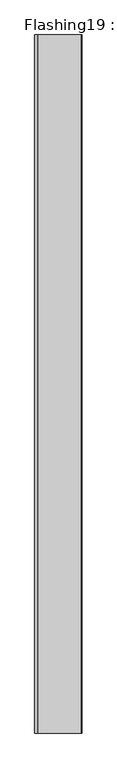
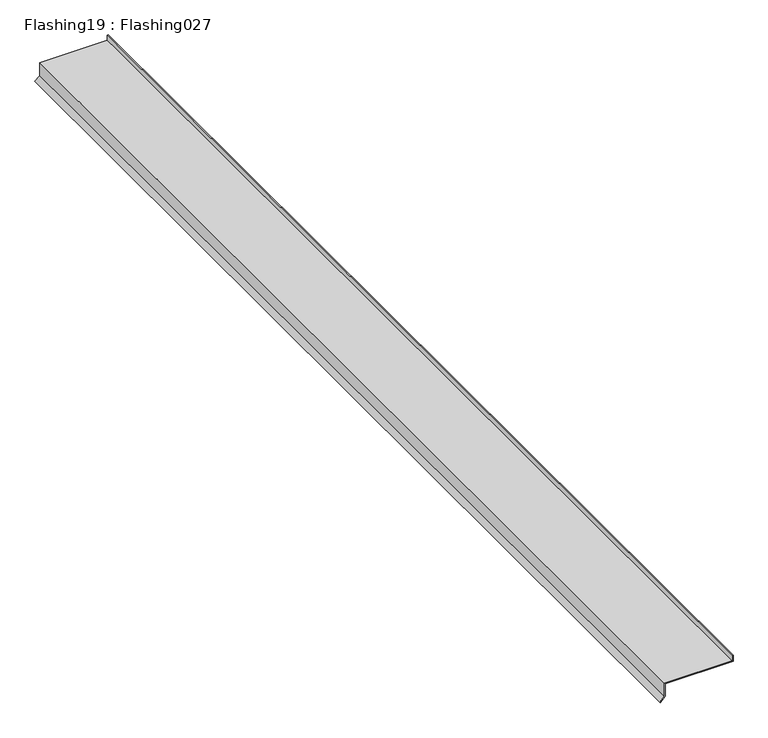
"""IFC4 building model written with IfcOpenShell, lengths in millimetres: proxy geometry, Flashing19 : Flashing027."""

import ifcopenshell
import ifcopenshell.guid

model = None  # the IFC model being written
_history = None  # IfcOwnerHistory: only IFC2X3 demands one
_inside = {}  # id of a spatial element -> (the spatial element, [elements in it])
_under = {}  # id of a project, library or spatial element -> (it, [spatial elements below it])
_declared = {}  # id of a project -> (the project, [libraries it declares])
_typed = {}  # id of a type object -> (the type object, [elements of that type])
_made_of = {}  # id of a material, layer set ... -> (it, [elements and type objects made of it])


def new_model(schema):
    """Start an empty IFC model of exactly this schema.

    Asked for "IFC4X3", IfcOpenShell would pick the latest addendum, in which some entities
    have other attributes; the version numbers below select the first issue.
    IFC2X3 requires an IfcOwnerHistory on every rooted entity: one is made here for all.
    """
    global model, _history
    if schema == "IFC4X3":
        model = ifcopenshell.file(schema_version=(4, 3, 0, 0))
    else:
        model = ifcopenshell.file(schema=schema)
    _inside.clear()
    _under.clear()
    _declared.clear()
    _typed.clear()
    _made_of.clear()
    _history = None
    if model.schema == "IFC2X3":
        org = make("IfcOrganization", Name="unknown")
        user = make(
            "IfcPersonAndOrganization",
            ThePerson=make("IfcPerson", FamilyName="unknown"),
            TheOrganization=org,
        )
        app = make(
            "IfcApplication",
            ApplicationDeveloper=org,
            Version="unknown",
            ApplicationFullName="unknown",
            ApplicationIdentifier="unknown",
        )
        _history = make(
            "IfcOwnerHistory",
            OwningUser=user,
            OwningApplication=app,
            ChangeAction="ADDED",
            CreationDate=0,
        )
    return model


def make(cls, **values):
    """One entity of the class cls with the attributes given. An attribute that is None is left unset."""
    return model.create_entity(
        cls, **{name: value for name, value in values.items() if value is not None}
    )


def rooted(cls, **values):
    """An entity with a GlobalId (a new one), such as an element, a storey or a relation."""
    return make(cls, GlobalId=ifcopenshell.guid.new(), OwnerHistory=_history, **values)


def si_unit(unit_type, name, prefix=None):
    """IfcSIUnit, for example si_unit("LENGTHUNIT", "METRE", prefix="MILLI")."""
    return make("IfcSIUnit", UnitType=unit_type, Prefix=prefix, Name=name)


def assignment(units):
    """IfcUnitAssignment: the units of a project."""
    return None if units is None else make("IfcUnitAssignment", Units=units)


def point(xyz):
    """IfcCartesianPoint."""
    return None if xyz is None else make("IfcCartesianPoint", Coordinates=xyz)


def direction(xyz):
    """IfcDirection."""
    return None if xyz is None else make("IfcDirection", DirectionRatios=xyz)


def frame(location, z_axis=None, x_axis=None):
    """IfcAxis2Placement3D, a coordinate frame: its origin and axes. An axis left out is left unset."""
    return make(
        "IfcAxis2Placement3D",
        Location=point(location),
        Axis=direction(z_axis),
        RefDirection=direction(x_axis),
    )


def origin():
    """The frame at (0, 0, 0) with its axes left unset."""
    return frame((0.0, 0.0, 0.0))


def place(relative_to, where):
    """IfcLocalPlacement: puts the frame where relative to a parent placement (None: the world)."""
    return make(
        "IfcLocalPlacement", PlacementRelTo=relative_to, RelativePlacement=where
    )


def context(
    kind, dimensions, precision=None, world=None, true_north=None, identifier=None
):
    """IfcGeometricRepresentationContext, for example the 3D "Model" context."""
    return make(
        "IfcGeometricRepresentationContext",
        ContextIdentifier=identifier,
        ContextType=kind,
        CoordinateSpaceDimension=dimensions,
        Precision=precision,
        WorldCoordinateSystem=world,
        TrueNorth=true_north,
    )


def project(units=None, contexts=None):
    """IfcProject with its units and contexts."""
    return rooted(
        "IfcProject",
        Name="project",
        RepresentationContexts=contexts,
        UnitsInContext=assignment(units),
    )


def spatial(cls, under=None, at=None, **own):
    """A site, building, storey or space (cls), placed at a placement, below another one or the project."""
    s = rooted(cls, ObjectPlacement=at, **own)
    if under is not None:
        _under.setdefault(under.id(), (under, []))[1].append(s)
    return s


def polyline(points):
    """IfcPolyline through the points."""
    return make("IfcPolyline", Points=[point(p) for p in points])


def outline(outer, holes=None, kind="AREA"):
    """IfcArbitraryClosedProfileDef: a profile drawn as a closed curve; with holes, ...WithVoids."""
    if holes is None:
        return make("IfcArbitraryClosedProfileDef", ProfileType=kind, OuterCurve=outer)
    return make(
        "IfcArbitraryProfileDefWithVoids",
        ProfileType=kind,
        OuterCurve=outer,
        InnerCurves=holes,
    )


def extrude(swept, where, along, depth):
    """IfcExtrudedAreaSolid: the profile swept, set in the frame where, extruded along a direction by depth."""
    return make(
        "IfcExtrudedAreaSolid",
        SweptArea=swept,
        Position=where,
        ExtrudedDirection=direction(along),
        Depth=depth,
    )


def shape(context_of_items, identifier, shape_type, items):
    """IfcShapeRepresentation: the items that make up one representation, for example the "Body"."""
    return make(
        "IfcShapeRepresentation",
        ContextOfItems=context_of_items,
        RepresentationIdentifier=identifier,
        RepresentationType=shape_type,
        Items=items,
    )


def source(mapping_origin, context_of_items, identifier, shape_type, items):
    """IfcRepresentationMap: a shape defined once, which mapped items show again and again."""
    return make(
        "IfcRepresentationMap",
        MappingOrigin=mapping_origin,
        MappedRepresentation=shape(context_of_items, identifier, shape_type, items),
    )


def transform(
    local_origin,
    x_axis=None,
    y_axis=None,
    z_axis=None,
    scale=None,
    scale2=None,
    scale3=None,
    uniform=True,
):
    """IfcCartesianTransformationOperator3D, or its non-uniform kind. x_axis, y_axis, z_axis: its Axis1, 2, 3."""
    if uniform:
        return make(
            "IfcCartesianTransformationOperator3D",
            Axis1=direction(x_axis),
            Axis2=direction(y_axis),
            LocalOrigin=point(local_origin),
            Scale=scale,
            Axis3=direction(z_axis),
        )
    return make(
        "IfcCartesianTransformationOperator3DnonUniform",
        Axis1=direction(x_axis),
        Axis2=direction(y_axis),
        LocalOrigin=point(local_origin),
        Scale=scale,
        Axis3=direction(z_axis),
        Scale2=scale2,
        Scale3=scale3,
    )


def mapped(mapping_source, mapping_target):
    """IfcMappedItem: shows the shape of a source again, moved by a transform."""
    return make(
        "IfcMappedItem", MappingSource=mapping_source, MappingTarget=mapping_target
    )


def made_of(thing, what):
    """Note that an element or type object is made of a material, layer set ...; save() writes the relation."""
    if what is not None:
        _made_of.setdefault(what.id(), (what, []))[1].append(thing)
    return thing


def element(
    cls,
    number,
    at=None,
    inside=None,
    cuts=None,
    type_object=None,
    material=None,
    context=None,
    identifier="Body",
    shape_type=None,
    held_by="IfcProductDefinitionShape",
    body=None,
    shapes=None,
    **own,
):
    """One element of the class cls, such as IfcWall. Its Tag is "e" and its number.

    at: its placement. inside: the storey or other place that contains it. cuts: it is an
    opening in that element (IfcRelVoidsElement). A single representation is given by context,
    identifier, shape_type and body (its items); several are given by shapes. held_by: the class
    of the entity that holds the representations. save() writes the other relations.
    """
    e = rooted(cls, Tag="e%d" % number, ObjectPlacement=at, **own)
    if body is not None:
        shapes = [shape(context, identifier, shape_type, body)]
    if shapes is not None:
        e.Representation = make(held_by, Representations=shapes)
    if inside is not None:
        _inside.setdefault(inside.id(), (inside, []))[1].append(e)
    if cuts is not None:
        rooted(
            "IfcRelVoidsElement", RelatingBuildingElement=cuts, RelatedOpeningElement=e
        )
    if type_object is not None:
        _typed.setdefault(type_object.id(), (type_object, []))[1].append(e)
    return made_of(e, material)


def aggregate(whole, parts):
    """IfcRelAggregates: a whole, such as a stair, and the parts it consists of."""
    return rooted("IfcRelAggregates", RelatingObject=whole, RelatedObjects=parts)


def save(model, path):
    """Write the relations noted so far, then the file.

    IfcRelAggregates (storeys below a building ...), IfcRelContainedInSpatialStructure (elements
    in a storey), IfcRelDefinesByType, IfcRelAssociatesMaterial and IfcRelDeclares: one each for
    every whole, place, type object, material and project.
    """
    for whole, parts in _under.values():
        aggregate(whole, parts)
    for where, things in _inside.values():
        rooted(
            "IfcRelContainedInSpatialStructure",
            RelatedElements=things,
            RelatingStructure=where,
        )
    for kind, things in _typed.values():
        rooted("IfcRelDefinesByType", RelatedObjects=things, RelatingType=kind)
    for what, things in _made_of.values():
        rooted("IfcRelAssociatesMaterial", RelatedObjects=things, RelatingMaterial=what)
    for by, libraries in _declared.values():
        rooted("IfcRelDeclares", RelatingContext=by, RelatedDefinitions=libraries)
    model.write(path)


def flashing19_flashing027_c57af108(model_context):
    return source(origin(), model_context, "Body", "SweptSolid", [
        extrude(outline(polyline([(40335.3398438, -986.5449829), (40325.640625, -986.5449829), (40325.640625, -1111.5771484), (40300.3872772, -1111.5771484), (40291.9157249, -1120.4555041), (40290.46875, -1119.0748291), (40299.53125, -1109.5771484), (40323.640625, -1109.5771484), (40323.640625, -984.5449829), (40335.3398438, -984.5449829), (40335.3398438, -986.5449829)])), frame((0.0, -1052.8906574, 0.0), z_axis=(0.0, 1.0, 0.0), x_axis=(0.0, 0.0, 1.0)), (0.0, 0.0, 1.0), 2000.0),
    ])


if __name__ == "__main__":
    model = new_model("IFC4")
    model_context = context("Model", 3, world=origin())
    ifc_project = project(units=[si_unit("LENGTHUNIT", "METRE", prefix="MILLI")], contexts=[model_context])
    site = spatial("IfcSite", under=ifc_project)
    building = spatial("IfcBuilding", under=site)
    placement = place(None, origin())
    flashing19_flashing027_shape = flashing19_flashing027_c57af108(model_context)
    element("IfcBuildingElementProxy", 1, Name="Flashing19 : Flashing027", ObjectType="Flashing19 : Flashing027", at=placement, inside=building, context=model_context, shape_type="MappedRepresentation", body=[
        mapped(flashing19_flashing027_shape, transform((0.0, 0.0, 0.0), x_axis=(1.0, 0.0, 0.0), y_axis=(0.0, 1.0, 0.0), z_axis=(0.0, 0.0, 1.0))),
    ])
    save(model, "model.ifc")

# Revit data of these elements
# Type "Flashing19 : Flashing027"
#   NameOverride = "Flashing027"
# Element 1 (IfcBuildingElementProxy, "Flashing19 : Flashing027")
#   Materials on its faces: "SILL PAN W/ END DAMS"
# Materials
#   "SILL PAN W/ END DAMS": class "Unassigned", colour RGB 255 170 255, transparency 0, Cost = 0
